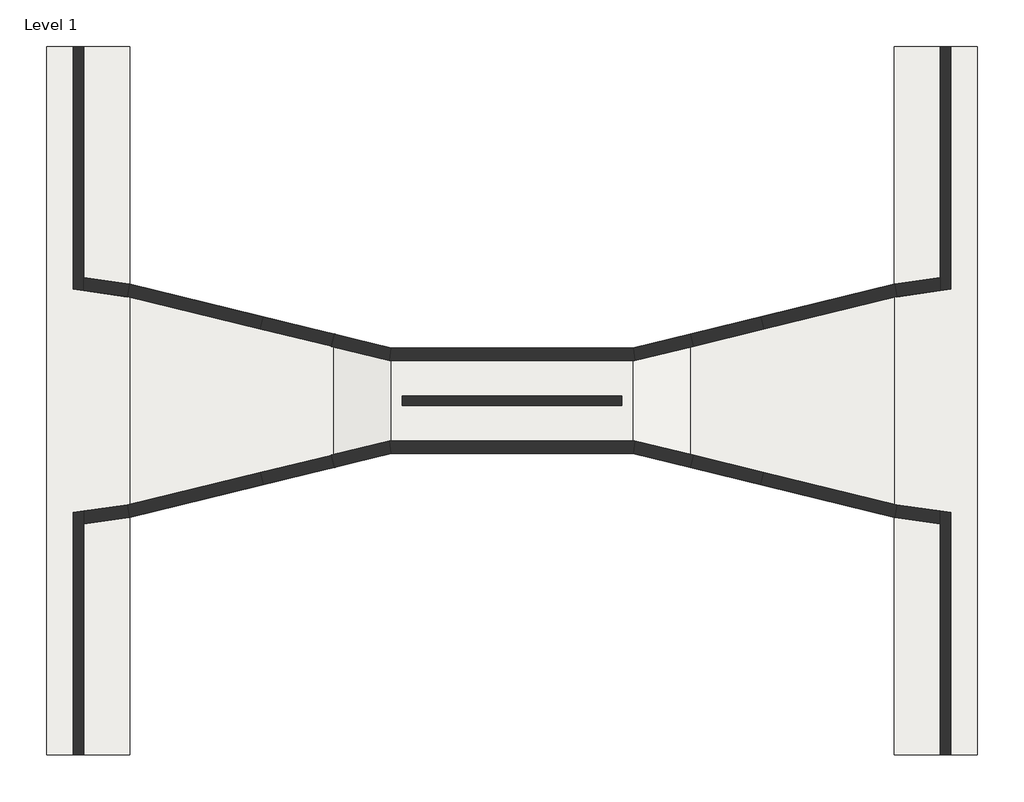
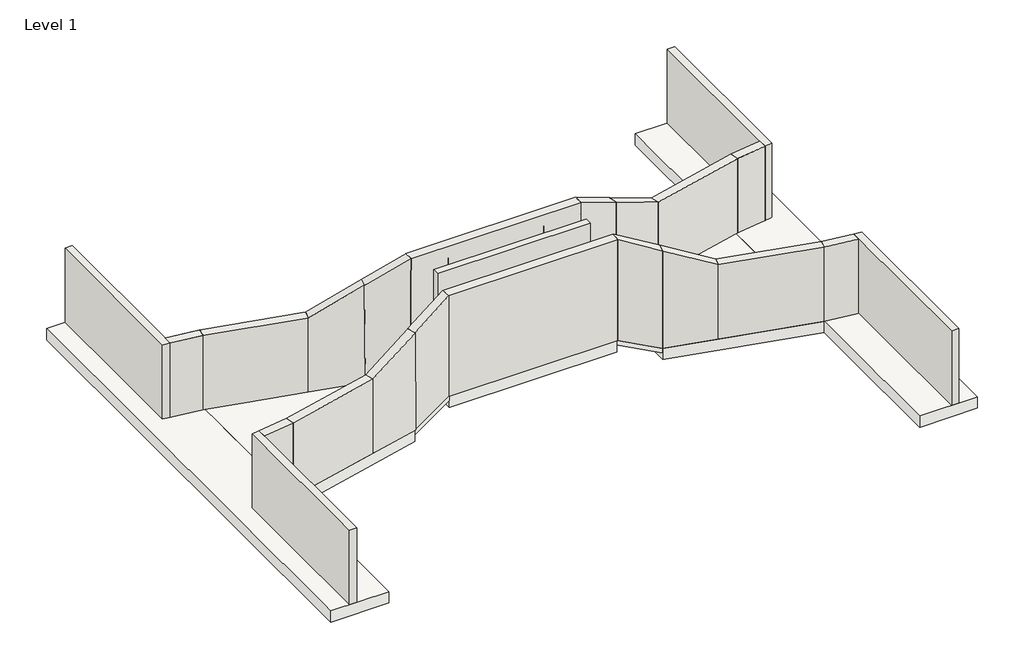
# One storey: 32 walls, 7 slabs.
"""IFC4 building model written with IfcOpenShell, lengths in millimetres."""

from ifc_helpers import new_model, si_unit, frame, origin, place, context, project, spatial, polyline, outline, extrude, faceted_brep, element, save

model = new_model("IFC4")

# Units and contexts
model_context = context("Model", 3, world=origin())
ifc_project = project(units=[si_unit("LENGTHUNIT", "METRE", prefix="MILLI")], contexts=[model_context])

# Site, building, storey
site = spatial("IfcSite", under=ifc_project)
building = spatial("IfcBuilding", under=site)
storey = spatial("IfcBuildingStorey", under=building, Name="Level 1", Elevation=0.0)

# Slabs
placement = place(None, origin())
element("IfcSlab", 1, ObjectType="Appronl", at=placement, inside=storey, context=model_context, shape_type="SweptSolid", body=[
    extrude(outline(polyline([(21800.0, -16601.0), (17901.0, -16601.0), (17901.0, 16601.0), (21800.0, 16601.0), (21800.0, -16601.0)])), frame((0.0, 0.0, -3600.0), z_axis=(0.0, 0.0, 1.0), x_axis=(1.0, 0.0, 0.0)), (0.0, 0.0, 1.0), 800.0),
])
element("IfcSlab", 2, ObjectType="Appronl", at=placement, inside=storey, context=model_context, shape_type="SweptSolid", body=[
    extrude(outline(polyline([(8350.0, 3127.0), (17901.0, 5458.0), (17901.0, -5458.0), (8350.0, -3127.0), (8350.0, 3127.0)])), frame((0.0, 0.0, -3600.0), z_axis=(0.0, 0.0, 1.0), x_axis=(1.0, 0.0, 0.0)), (0.0, 0.0, 1.0), 800.0),
])
element("IfcSlab", 3, ObjectType="Appronl", at=placement, inside=storey, context=model_context, shape_type="SweptSolid", body=[
    extrude(outline(polyline([(-21800.0, 16601.0), (-17901.0, 16601.0), (-17901.0, -16601.0), (-21800.0, -16601.0), (-21800.0, 16601.0)])), frame((0.0, 0.0, -3600.0), z_axis=(0.0, 0.0, 1.0), x_axis=(1.0, 0.0, 0.0)), (0.0, 0.0, 1.0), 800.0),
])
element("IfcSlab", 4, ObjectType="Appronl", at=placement, inside=storey, context=model_context, shape_type="SweptSolid", body=[
    extrude(outline(polyline([(-8350.0, 3127.0), (-8350.0, -3127.0), (-17901.0, -5458.0), (-17901.0, 5458.0), (-8350.0, 3127.0)])), frame((0.0, 0.0, -3600.0), z_axis=(0.0, 0.0, 1.0), x_axis=(1.0, 0.0, 0.0)), (0.0, 0.0, 1.0), 800.0),
])
element("IfcSlab", 5, ObjectType="Appronl", at=placement, inside=storey, context=model_context, shape_type="SweptSolid", body=[
    extrude(outline(polyline([(5650.0, 2468.0), (5650.0, -2468.0), (-5650.0, -2468.0), (-5650.0, 2468.0), (5650.0, 2468.0)])), frame((0.0, 0.0, -2500.0), z_axis=(0.0, 0.0, 1.0), x_axis=(1.0, 0.0, 0.0)), (0.0, 0.0, 1.0), 800.0),
])
element("IfcSlab", 6, ObjectType="Generic - 12\"", at=placement, inside=storey, context=model_context, shape_type="Brep", body=[
    faceted_brep([(-5650.0, 2468.0, -2029.1248403), (-5650.0, -2468.0, -2029.1248403), (-8350.0, -3127.0, -3129.1248403), (-8350.0, 3127.0, -3129.1248403), (-5650.0, 2468.0, -1700.0), (-8350.0, 3127.0, -2800.0), (-8350.0, -3127.0, -2800.0), (-5650.0, -2468.0, -1700.0)], [[[0, 1, 2, 3]], [[4, 5, 6, 7]], [[1, 0, 4, 7]], [[2, 1, 7, 6]], [[3, 2, 6, 5]], [[0, 3, 5, 4]]]),
])
element("IfcSlab", 7, ObjectType="Generic - 12\"", at=placement, inside=storey, context=model_context, shape_type="Brep", body=[
    faceted_brep([(5650.0, 2468.0, -2029.1248403), (8350.0, 3127.0, -3129.1248403), (8350.0, -3127.0, -3129.1248403), (5650.0, -2468.0, -2029.1248403), (5650.0, 2468.0, -1700.0), (5650.0, -2468.0, -1700.0), (8350.0, -3127.0, -2800.0), (8350.0, 3127.0, -2800.0)], [[[0, 1, 2, 3]], [[4, 5, 6, 7]], [[1, 0, 4, 7]], [[2, 1, 7, 6]], [[3, 2, 6, 5]], [[0, 3, 5, 4]]]),
])

# Walls
element("IfcWall", 8, ObjectType="Wingwall", at=placement, inside=storey, context=model_context, shape_type="SweptSolid", body=[
    extrude(outline(polyline([(-20050.0, 5767.2805137), (-17916.0428831, 5461.9054729), (-18029.9571169, 4872.0945271), (-20050.0, 5161.1681326), (-20050.0, 5767.2805137)])), frame((0.0, 0.0, -2800.0), z_axis=(0.0, 0.0, 1.0), x_axis=(1.0, 0.0, 0.0)), (0.0, 0.0, 1.0), 5300.0),
])
element("IfcWall", 9, ObjectType="Wingwall", at=placement, inside=storey, context=model_context, shape_type="SweptSolid", body=[
    extrude(outline(polyline([(-11792.4456337, 3349.3873565), (-18029.9571169, 4872.0945271), (-17916.0428831, 5461.9054729), (-11651.5543663, 3932.6126435), (-11792.4456337, 3349.3873565)])), frame((0.0, 0.0, -2800.0), z_axis=(0.0, 0.0, 1.0), x_axis=(1.0, 0.0, 0.0)), (0.0, 0.0, 1.0), 5300.0),
])
element("IfcWall", 10, ObjectType="Wingwall", at=placement, inside=storey, context=model_context, shape_type="Brep", body=[
    faceted_brep([(-11651.5543663, 3932.6126435, -2800.0), (-11651.5543663, 3932.6126435, 2500.3510698), (-8352.2565059, 3143.9904385, 4150.0), (-8280.2565059, 3126.780474, -2800.0), (-11792.4456336, 3349.3873565, -2800.0), (-8419.7434941, 2543.219526, -2800.0), (-8491.7434941, 2560.4294904, 4150.0), (-11792.4456336, 3349.3873565, 2499.6489302)], [[[0, 1, 2, 3]], [[4, 5, 6, 7]], [[2, 1, 7, 6]], [[3, 2, 6, 5]], [[0, 3, 5, 4]], [[1, 0, 4, 7]]]),
])
element("IfcWall", 11, ObjectType="Wingwall", at=placement, inside=storey, context=model_context, shape_type="Brep", body=[
    faceted_brep([(-8350.8659334, 3126.4445823, 4150.0), (-5685.9184792, 2476.0, 5482.4737271), (-5685.9184792, 2476.0, -1714.671918), (-8278.8659334, 3108.871249, -2800.0), (-8493.1340666, 2543.5554177, 4150.0), (-8421.1340666, 2525.9820843, -2800.0), (-5758.0815208, 1876.0, -1685.328082), (-5758.0815208, 1876.0, 5517.5262729)], [[[0, 1, 2, 3]], [[4, 5, 6, 7]], [[1, 0, 4, 7]], [[3, 2, 6, 5]], [[0, 3, 5, 4]], [[1, 7, 6, 2]]]),
])
element("IfcWall", 12, ObjectType="Wingwall", at=placement, inside=storey, context=model_context, shape_type="Brep", body=[
    faceted_brep([(5685.9184792, 2476.0, -1714.2806668), (5685.9184792, 2476.0, 5482.4737271), (8350.8659334, 3126.4445823, 4150.0), (8350.8659334, 3126.4445823, -2800.0), (5758.0815208, 1876.0, 5517.5262729), (5758.0815208, 1876.0, -1685.7193332), (8493.1340666, 2543.5554177, -2800.0), (8493.1340666, 2543.5554177, 4150.0)], [[[0, 1, 2, 3]], [[4, 5, 6, 7]], [[2, 1, 4, 7]], [[0, 3, 6, 5]], [[2, 7, 6, 3]], [[0, 5, 4, 1]]]),
])
element("IfcWall", 13, ObjectType="Wingwall", at=placement, inside=storey, context=model_context, shape_type="SweptSolid", body=[
    extrude(outline(polyline([(18029.9571169, 4872.0945271), (11793.1469574, 3349.5585643), (11650.8530426, 3932.4414357), (17916.0428831, 5461.9054729), (18029.9571169, 4872.0945271)])), frame((0.0, 0.0, -2800.0), z_axis=(0.0, 0.0, 1.0), x_axis=(1.0, 0.0, 0.0)), (0.0, 0.0, 1.0), 5300.0),
])
element("IfcWall", 14, ObjectType="Wingwall", at=placement, inside=storey, context=model_context, shape_type="SweptSolid", body=[
    extrude(outline(polyline([(17916.0428831, 5461.9054729), (20050.0, 5767.2805137), (20050.0, 5161.1681326), (18029.9571169, 4872.0945271), (17916.0428831, 5461.9054729)])), frame((0.0, 0.0, -2800.0), z_axis=(0.0, 0.0, 1.0), x_axis=(1.0, 0.0, 0.0)), (0.0, 0.0, 1.0), 5300.0),
])
element("IfcWall", 15, ObjectType="Wingwall", at=placement, inside=storey, context=model_context, shape_type="SweptSolid", body=[
    extrude(outline(polyline([(5300.0, 0.0), (6950.0, -3397.0039741), (0.0, -3397.0039741), (0.0, 0.0), (5300.0, 0.0)])), frame((11793.1803701, 3349.566723, -2800.0), z_axis=(-0.23726790022826785, 0.9714442565177216, 0.0), x_axis=(0.0, 0.0, 1.0)), (0.0, 0.0, 1.0), 600.0),
])
element("IfcWall", 16, ObjectType="Wingwall", at=placement, inside=storey, context=model_context, shape_type="SweptSolid", body=[
    extrude(outline(polyline([(-20050.0, -5161.1681326), (-18029.9571169, -4872.0945271), (-17916.0428831, -5461.9054729), (-20050.0, -5767.2805137), (-20050.0, -5161.1681326)])), frame((0.0, 0.0, -2800.0), z_axis=(0.0, 0.0, 1.0), x_axis=(1.0, 0.0, 0.0)), (0.0, 0.0, 1.0), 5300.0),
])
element("IfcWall", 17, ObjectType="Wingwall", at=placement, inside=storey, context=model_context, shape_type="SweptSolid", body=[
    extrude(outline(polyline([(-11651.5543663, -3932.6126435), (-17916.0428831, -5461.9054729), (-18029.9571169, -4872.0945271), (-11792.4456337, -3349.3873565), (-11651.5543663, -3932.6126435)])), frame((0.0, 0.0, -2800.0), z_axis=(0.0, 0.0, 1.0), x_axis=(1.0, 0.0, 0.0)), (0.0, 0.0, 1.0), 5300.0),
])
element("IfcWall", 18, ObjectType="Wingwall", at=placement, inside=storey, context=model_context, shape_type="Brep", body=[
    faceted_brep([(-11792.4456336, -3349.3873565, -2800.0), (-11792.4456336, -3349.3873565, 2499.6489302), (-8491.7434941, -2560.4294904, 4150.0), (-8419.7434941, -2543.219526, -2800.0), (-11651.5543663, -3932.6126435, -2800.0), (-8280.2565059, -3126.780474, -2800.0), (-8352.2565059, -3143.9904385, 4150.0), (-11651.5543663, -3932.6126435, 2500.3510698)], [[[0, 1, 2, 3]], [[4, 5, 6, 7]], [[2, 1, 7, 6]], [[3, 2, 6, 5]], [[0, 3, 5, 4]], [[1, 0, 4, 7]]]),
])
element("IfcWall", 19, ObjectType="Wingwall", at=placement, inside=storey, context=model_context, shape_type="Brep", body=[
    faceted_brep([(-8493.1340666, -2543.5554177, 4150.0), (-5758.0815208, -1876.0, 5517.5262729), (-5758.0815208, -1876.0, -1685.328082), (-8421.1340666, -2525.9820843, -2800.0), (-8350.8659334, -3126.4445823, 4150.0), (-8278.8659334, -3108.871249, -2800.0), (-5685.9184792, -2476.0, -1714.671918), (-5685.9184792, -2476.0, 5482.4737271)], [[[0, 1, 2, 3]], [[4, 5, 6, 7]], [[1, 0, 4, 7]], [[3, 2, 6, 5]], [[0, 3, 5, 4]], [[2, 1, 7, 6]]]),
])
element("IfcWall", 20, ObjectType="Wingwall", at=placement, inside=storey, context=model_context, shape_type="Brep", body=[
    faceted_brep([(5758.0815208, -1876.0, -1685.7193332), (5758.0815208, -1876.0, 5517.5262729), (8493.1340666, -2543.5554177, 4150.0), (8493.1340666, -2543.5554177, -2800.0), (5685.9184792, -2476.0, -1714.2806668), (8350.8659334, -3126.4445823, -2800.0), (8350.8659334, -3126.4445823, 4150.0), (5685.9184792, -2476.0, 5482.4737271)], [[[0, 1, 2, 3]], [[4, 5, 6, 7]], [[2, 1, 7, 6]], [[3, 2, 6, 5]], [[0, 3, 5, 4]], [[1, 0, 4, 7]]]),
])
element("IfcWall", 21, ObjectType="Wingwall", at=placement, inside=storey, context=model_context, shape_type="SweptSolid", body=[
    extrude(outline(polyline([(5300.0, 0.0), (6950.0, -3397.0039741), (0.0, -3397.0039741), (0.0, 0.0), (5300.0, 0.0)])), frame((11650.8196299, -3932.433277, -2800.0), z_axis=(0.23726790022826785, 0.9714442565177216, 0.0), x_axis=(0.0, 0.0, 1.0)), (0.0, 0.0, 1.0), 600.0),
])
element("IfcWall", 22, ObjectType="Wingwall", at=placement, inside=storey, context=model_context, shape_type="SweptSolid", body=[
    extrude(outline(polyline([(17916.0428831, -5461.9054729), (11650.8530426, -3932.4414357), (11793.1469574, -3349.5585643), (18029.9571169, -4872.0945271), (17916.0428831, -5461.9054729)])), frame((0.0, 0.0, -2800.0), z_axis=(0.0, 0.0, 1.0), x_axis=(1.0, 0.0, 0.0)), (0.0, 0.0, 1.0), 5300.0),
])
element("IfcWall", 23, ObjectType="Wingwall", at=placement, inside=storey, context=model_context, shape_type="SweptSolid", body=[
    extrude(outline(polyline([(18029.9571169, -4872.0945271), (20050.0, -5161.1681326), (20050.0, -5767.2805137), (17916.0428831, -5461.9054729), (18029.9571169, -4872.0945271)])), frame((0.0, 0.0, -2800.0), z_axis=(0.0, 0.0, 1.0), x_axis=(1.0, 0.0, 0.0)), (0.0, 0.0, 1.0), 5300.0),
])
element("IfcWall", 24, ObjectType="Wingwall", at=placement, inside=storey, context=model_context, shape_type="SweptSolid", body=[
    extrude(outline(polyline([(-20050.0, 5767.2805137), (-17930.5021265, 5463.9746298), (-18015.4978735, 4870.0253702), (-20050.0, 5161.1681326), (-20050.0, 5767.2805137)])), frame((0.0, 0.0, -2800.0), z_axis=(0.0, 0.0, 1.0), x_axis=(1.0, 0.0, 0.0)), (0.0, 0.0, 1.0), 5300.0),
])
element("IfcWall", 25, ObjectType="Wingwall", at=placement, inside=storey, context=model_context, shape_type="SweptSolid", body=[
    extrude(outline(polyline([(-11793.1469574, 3349.5585643), (-18029.9571169, 4872.0945271), (-17916.0428831, 5461.9054729), (-11650.8530426, 3932.4414357), (-11793.1469574, 3349.5585643)])), frame((0.0, 0.0, -2800.0), z_axis=(0.0, 0.0, 1.0), x_axis=(1.0, 0.0, 0.0)), (0.0, 0.0, 1.0), 5300.0),
])
element("IfcWall", 26, ObjectType="Wingwall", at=placement, inside=storey, context=model_context, shape_type="Brep", body=[
    faceted_brep([(-11651.5543663, 3932.6126435, -2800.0), (-11651.5543663, 3932.6126435, 2500.3510698), (-8352.2565059, 3143.9904385, 4150.0), (-8280.2565059, 3126.780474, -2800.0), (-11792.4456336, 3349.3873565, -2800.0), (-8419.7434941, 2543.219526, -2800.0), (-8491.7434941, 2560.4294904, 4150.0), (-11792.4456336, 3349.3873565, 2499.6489302)], [[[0, 1, 2, 3]], [[4, 5, 6, 7]], [[2, 1, 7, 6]], [[3, 2, 6, 5]], [[0, 3, 5, 4]], [[1, 0, 4, 7]]]),
])
element("IfcWall", 27, ObjectType="Wingwall", at=placement, inside=storey, context=model_context, shape_type="Brep", body=[
    faceted_brep([(-8350.8659334, 3126.4445823, 4150.0), (-5685.9184792, 2476.0, 5482.4737271), (-5685.9184792, 2476.0, -1714.671918), (-8278.8659334, 3108.871249, -2800.0), (-8493.1340666, 2543.5554177, 4150.0), (-8421.1340666, 2525.9820843, -2800.0), (-5758.0815208, 1876.0, -1685.328082), (-5758.0815208, 1876.0, 5517.5262729)], [[[0, 1, 2, 3]], [[4, 5, 6, 7]], [[1, 0, 4, 7]], [[3, 2, 6, 5]], [[0, 3, 5, 4]], [[1, 7, 6, 2]]]),
])
element("IfcWall", 28, ObjectType="Wingwall", at=placement, inside=storey, context=model_context, shape_type="Brep", body=[
    faceted_brep([(5685.9184792, 2476.0, -1714.2806668), (5685.9184792, 2476.0, 5482.4737271), (8350.8659334, 3126.4445823, 4150.0), (8350.8659334, 3126.4445823, -2800.0), (5758.0815208, 1876.0, 5517.5262729), (5758.0815208, 1876.0, -1685.7193332), (8493.1340666, 2543.5554177, -2800.0), (8493.1340666, 2543.5554177, 4150.0)], [[[0, 1, 2, 3]], [[4, 5, 6, 7]], [[2, 1, 4, 7]], [[0, 3, 6, 5]], [[0, 5, 4, 1]], [[2, 7, 6, 3]]]),
])
element("IfcWall", 29, ObjectType="Wingwall", at=placement, inside=storey, context=model_context, shape_type="SweptSolid", body=[
    extrude(outline(polyline([(5300.0, 0.0), (6950.0, -3397.0039741), (0.0, -3397.0039741), (0.0, 0.0), (5300.0, 0.0)])), frame((11793.1803701, 3349.566723, -2800.0), z_axis=(-0.23726790022826785, 0.9714442565177216, 0.0), x_axis=(0.0, 0.0, 1.0)), (0.0, 0.0, 1.0), 600.0),
])
element("IfcWall", 30, ObjectType="Wingwall", at=placement, inside=storey, context=model_context, shape_type="SweptSolid", body=[
    extrude(outline(polyline([(18029.9571169, 4872.0945271), (11793.1469574, 3349.5585643), (11650.8530426, 3932.4414357), (17916.0428831, 5461.9054729), (18029.9571169, 4872.0945271)])), frame((0.0, 0.0, -2800.0), z_axis=(0.0, 0.0, 1.0), x_axis=(1.0, 0.0, 0.0)), (0.0, 0.0, 1.0), 5300.0),
])
element("IfcWall", 31, ObjectType="Wingwall", at=placement, inside=storey, context=model_context, shape_type="SweptSolid", body=[
    extrude(outline(polyline([(17930.5021265, 5463.9746298), (20050.0, 5767.2805137), (20050.0, 5161.1681326), (18015.4978735, 4870.0253702), (17930.5021265, 5463.9746298)])), frame((0.0, 0.0, -2800.0), z_axis=(0.0, 0.0, 1.0), x_axis=(1.0, 0.0, 0.0)), (0.0, 0.0, 1.0), 5300.0),
])
element("IfcWall", 32, ObjectType="Abutment", at=placement, inside=storey, context=model_context, shape_type="Brep", body=[
    faceted_brep([(-5758.0815208, 1876.0, -1700.0), (5758.0815208, 1876.0, -1700.0), (5758.0815208, 1876.0, 4673.4903305), (5722.0, 1876.0, 4673.4903305), (5722.0, 1876.0, 5500.0), (-5722.0, 1876.0, 5500.0), (-5722.0, 1876.0, 4673.4903305), (-5758.0815208, 1876.0, 4673.4903305), (-5685.9184792, 2476.0, -1700.0), (-5685.9184792, 2476.0, 4673.4903305), (-5722.0, 2476.0, 4673.4903305), (-5722.0, 2476.0, 5500.0), (5722.0, 2476.0, 5500.0), (5722.0, 2476.0, 4673.4903305), (5685.9184792, 2476.0, 4673.4903305), (5685.9184792, 2476.0, -1700.0), (-5722.0, 2176.0, 4673.4903305), (5722.0, 2176.0, 4673.4903305)], [[[0, 1, 2, 3, 4, 5, 6, 7]], [[8, 9, 10, 11, 12, 13, 14, 15]], [[1, 0, 8, 15]], [[5, 4, 12, 11]], [[6, 5, 11, 10, 16]], [[6, 16, 7]], [[0, 7, 16, 9, 8]], [[16, 10, 9]], [[4, 3, 17, 13, 12]], [[13, 17, 14]], [[2, 1, 15, 14, 17]], [[17, 3, 2]]]),
])
element("IfcWall", 33, ObjectType="Abutment", at=placement, inside=storey, context=model_context, shape_type="SweptSolid", body=[
    extrude(outline(polyline([(5685.9184792, -2476.0), (-5685.9184792, -2476.0), (-5758.0815208, -1876.0), (5758.0815208, -1876.0), (5685.9184792, -2476.0)])), frame((0.0, 0.0, -1700.0), z_axis=(0.0, 0.0, 1.0), x_axis=(1.0, 0.0, 0.0)), (0.0, 0.0, 1.0), 7200.0),
])
element("IfcWall", 34, ObjectType="Abutment", at=placement, inside=storey, context=model_context, shape_type="Brep", body=[
    faceted_brep([(-3227.648373, 1876.0, -1700.0), (3227.648373, 1876.0, -1700.0), (3227.648373, 1876.0, 4673.4903305), (5722.0, 1876.0, 4673.4903305), (5722.0, 1876.0, 5500.0), (-5722.0, 1876.0, 5500.0), (-5722.0, 1876.0, 4673.4903305), (-3227.648373, 1876.0, 4673.4903305), (-5685.9184792, 2476.0, -1700.0), (-5685.9184792, 2476.0, 4673.4903305), (-5722.0, 2476.0, 4673.4903305), (-5722.0, 2476.0, 5500.0), (5722.0, 2476.0, 5500.0), (5722.0, 2476.0, 4673.4903305), (5685.9184792, 2476.0, 4673.4903305), (5685.9184792, 2476.0, -1700.0)], [[[0, 1, 2, 3, 4, 5, 6, 7]], [[8, 9, 10, 11, 12, 13, 14, 15]], [[1, 0, 8, 15]], [[5, 4, 12, 11]], [[6, 5, 11, 10]], [[6, 10, 9, 7]], [[0, 7, 9, 8]], [[4, 3, 13, 12]], [[13, 3, 2, 14]], [[2, 1, 15, 14]]]),
])
element("IfcWall", 35, ObjectType="Pier", at=placement, inside=storey, context=model_context, shape_type="SweptSolid", body=[
    extrude(outline(polyline([(5150.0, -225.0), (-5150.0, -225.0), (-5150.0, 225.0), (5150.0, 225.0), (5150.0, -225.0)])), frame((0.0, 0.0, -1700.0), z_axis=(0.0, 0.0, 1.0), x_axis=(1.0, 0.0, 0.0)), (0.0, 0.0, 1.0), 7200.0),
])
element("IfcWall", 36, ObjectType="Return Wall", at=placement, inside=storey, context=model_context, shape_type="Brep", body=[
    faceted_brep([(20550.0, 5232.7194863, -2800.0), (20550.0, 16601.0, -2800.0), (20550.0, 16601.0, 2500.0), (20550.0, 5232.7194863, 2500.0), (20050.0, 5161.1681326, -2800.0), (20050.0, 5161.1681326, 2500.0), (20050.0, 5767.2805137, 2500.0), (20050.0, 16601.0, 2500.0), (20050.0, 16601.0, -2800.0), (20050.0, 5767.2805137, -2800.0)], [[[0, 1, 2, 3]], [[4, 5, 6, 7, 8, 9]], [[1, 0, 4, 9, 8]], [[2, 1, 8, 7]], [[3, 2, 7, 6, 5]], [[0, 3, 5, 4]]]),
])
element("IfcWall", 37, ObjectType="Return Wall", at=placement, inside=storey, context=model_context, shape_type="Brep", body=[
    faceted_brep([(20550.0, -16601.0, -2800.0), (20550.0, -5232.7194863, -2800.0), (20550.0, -5232.7194863, 2500.0), (20550.0, -16601.0, 2500.0), (20050.0, -16601.0, -2800.0), (20050.0, -16601.0, 2500.0), (20050.0, -5767.2805137, 2500.0), (20050.0, -5161.1681326, 2500.0), (20050.0, -5161.1681326, -2800.0), (20050.0, -5767.2805137, -2800.0)], [[[0, 1, 2, 3]], [[4, 5, 6, 7, 8, 9]], [[1, 0, 4, 9, 8]], [[3, 2, 7, 6, 5]], [[0, 3, 5, 4]], [[2, 1, 8, 7]]]),
])
element("IfcWall", 38, ObjectType="Return Wall", at=placement, inside=storey, context=model_context, shape_type="Brep", body=[
    faceted_brep([(-20050.0, -16601.0, -2800.0), (-20050.0, -5767.2805137, -2800.0), (-20050.0, -5161.1681326, -2800.0), (-20050.0, -5161.1681326, 2500.0), (-20050.0, -5767.2805137, 2500.0), (-20050.0, -16601.0, 2500.0), (-20550.0, -16601.0, -2800.0), (-20550.0, -16601.0, 2500.0), (-20550.0, -5232.7194863, 2500.0), (-20550.0, -5232.7194863, -2800.0)], [[[0, 1, 2, 3, 4, 5]], [[6, 7, 8, 9]], [[2, 1, 0, 6, 9]], [[5, 4, 3, 8, 7]], [[0, 5, 7, 6]], [[3, 2, 9, 8]]]),
])
element("IfcWall", 39, ObjectType="Return Wall", at=placement, inside=storey, context=model_context, shape_type="Brep", body=[
    faceted_brep([(-20050.0, 5161.1681326, -2800.0), (-20050.0, 5767.2805137, -2800.0), (-20050.0, 16601.0, -2800.0), (-20050.0, 16601.0, 2500.0), (-20050.0, 5767.2805137, 2500.0), (-20050.0, 5161.1681326, 2500.0), (-20550.0, 5232.7194863, -2800.0), (-20550.0, 5232.7194863, 2500.0), (-20550.0, 16601.0, 2500.0), (-20550.0, 16601.0, -2800.0)], [[[0, 1, 2, 3, 4, 5]], [[6, 7, 8, 9]], [[2, 1, 0, 6, 9]], [[3, 2, 9, 8]], [[5, 4, 3, 8, 7]], [[0, 5, 7, 6]]]),
])

save(model, "model.ifc")

# Revit data of these elements
# Project information
#   Project Issue Date = "Issue Date"
#   Project Status = "Project Status"
#   Client Name = "Owner"
#   Project Address = "Enter address here"
#   Project Name = "Project Name"
#   Project Number = "Project Number"
# Type "Appronl"
#   Assembly Code = "B1010"
#   Function = 0
#   Layers, outside or top first: 2' - 7.49606" "CONCR" (function 1)
# Type "Generic - 12\""
#   Assembly Code = "B1010"
#   Function = 0
#   Layers, outside or top first: 1' - 0" no material (function 1)
# Type "Wingwall"
#   Assembly Code = "B2010"
#   Layers, outside or top first: 1' - 11.62205" "CONCR" (function 1)
# Type "Abutment"
#   Assembly Code = "B2010"
#   Layers, outside or top first: 1' - 11.62205" "CONCR" (function 1)
# Type "Pier"
#   Assembly Code = "B2010"
#   Layers, outside or top first: 1' - 5.71654" "CONCR" (function 1)
# Type "Return Wall"
#   Assembly Code = "B2010"
#   Layers, outside or top first: 1' - 7.68504" "CONCR" (function 1)
# Elements 1, 2, 3, 4 (IfcSlab, "Appronl")
#   Height Offset From Level = -9' - 2.23622"
#   built-in parameter 1001954 = 1
#   Phase Created = New Construction
#   Materials on its faces: "CONCR"
# Element 5 (IfcSlab, "Appronl")
#   Height Offset From Level = -5' - 6.92913"
#   built-in parameter 1001954 = 1
#   Phase Created = New Construction
#   Materials on its faces: "CONCR"
# Elements 6, 7 (IfcSlab, "Generic - 12\"")
#   Height Offset From Level = -9' - 2.23622"
#   built-in parameter 1001954 = 1
#   Phase Created = New Construction
#   Materials on its faces: "Default Floor"
# Elements 8, 9, 13, 14, 16, 17, 22, 23, 24, 25, 30, 31 (IfcWall, "Wingwall")
#   built-in parameter 1001111 = -9' - 2.23622"
#   Top Offset = -1' - 9.5748"
#   Base Offset = -9' - 2.23622"
#   Unconnected Height = 17' - 4.66142"
#   wall height = 17' - 4.66142"
#   Phase Created = New Construction
#   Base Constraint = Level 1
#   Top Constraint = Level 2
#   Materials on its faces: "CONCR"
# Elements 10, 15, 18, 21, 26, 29 (IfcWall, "Wingwall")
#   built-in parameter 1001111 = -9' - 2.23622"
#   Top Offset = 3' - 7.38583"
#   Base Offset = -9' - 2.23622"
#   Unconnected Height = 22' - 9.62205"
#   wall height = 22' - 9.62205"
#   Phase Created = New Construction
#   Base Constraint = Level 1
#   Top Constraint = Level 2
#   Materials on its faces: "CONCR"
# Elements 11, 12, 19, 20, 27, 28 (IfcWall, "Wingwall")
#   built-in parameter 1001111 = -9' - 2.23622"
#   Top Offset = 8' - 0.53543"
#   Base Offset = -9' - 2.23622"
#   Unconnected Height = 27' - 2.77165"
#   wall height = 27' - 2.77165"
#   Phase Created = New Construction
#   Base Constraint = Level 1
#   Top Constraint = Level 2
#   Materials on its faces: "CONCR"
# Elements 32, 33, 34 (IfcWall, "Abutment")
#   built-in parameter 1001111 = -5' - 6.92913"
#   Top Offset = 8' - 0.53543"
#   Base Offset = -5' - 6.92913"
#   Unconnected Height = 23' - 7.46457"
#   wall height = 23' - 7.46457"
#   Phase Created = New Construction
#   Base Constraint = Level 1
#   Top Constraint = Level 2
#   Materials on its faces: "CONCR"
# Element 35 (IfcWall, "Pier")
#   built-in parameter 1001111 = -5' - 6.92913"
#   Top Offset = 8' - 0.53543"
#   Base Offset = -5' - 6.92913"
#   Unconnected Height = 23' - 7.46457"
#   wall height = 23' - 7.46457"
#   Phase Created = New Construction
#   Base Constraint = Level 1
#   Top Constraint = Level 2
#   Materials on its faces: "CONCR"
# Elements 36, 37, 38, 39 (IfcWall, "Return Wall")
#   built-in parameter 1001111 = -9' - 2.23622"
#   Top Offset = -1' - 9.5748"
#   Base Offset = -9' - 2.23622"
#   Unconnected Height = 17' - 4.66142"
#   wall height = 17' - 4.66142"
#   Phase Created = New Construction
#   Base Constraint = Level 1
#   Top Constraint = Level 2
#   Materials on its faces: "CONCR"
# Materials
#   "CONCR": class "Unassigned", colour RGB 192 192 192, transparency 0
#   "Default Floor": class "Miscellaneous", colour RGB 128 128 128, transparency 0, Cost = 0
